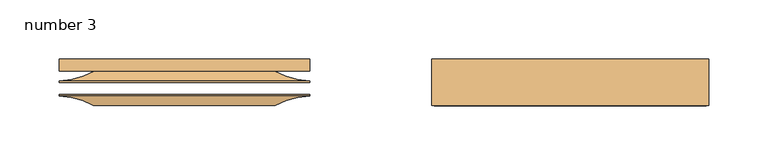
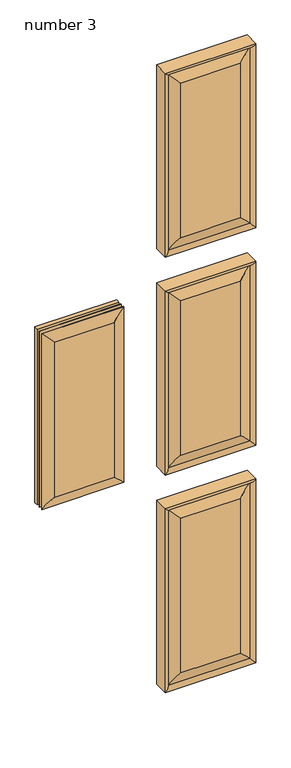
# IFC4 building model written with IfcOpenShell, lengths in millimetres: door geometry, Door-Interior-Karona-K5660-6_Panel : number 3.
# Revit data of these elements (continued)
# Type "Door-Interior-Karona-K5660-6_Panel : number 3" (continued)
#   Bottom Rail Height = 0' - 8 1/2"
#   3D Open Angle = 0.00°
#   Thickness = 0' - 1 3/4"
#   Stop Thickness = 0' - 0 1/2"
#   Stop Depth = 0' - 1 3/8"
#   Rough Width = 2' - 9 29/32"
#   Rough Height = 6' - 8 61/64"
#   Rabbet Width = 0' - 1 3/4"
#   Jamb Offset = 0' - 0 61/64"
#   Hinge Offset = 0' - 0 3/4"
#   Jamb Thickness = 0' - 0 29/32"
#   Ext. Frame Thickness = 0' - 0 5/8"
#   Int. Frame Thickness = 0' - 0 5/8"
#   Height = 6' - 8"
#   Width = 2' - 8"
#   3D Angle = 0.00°
#   Trim Visible = yes
#   Square Sticking Profile = no
#   Raised Panel Door = yes
#   Ovolo Sticking Profile = yes
#   Ogee Sticking Profile = no
#   Mission Sticking Profile = no
#   Hinge Visible = yes
#   Glass Panel Door = no
#   Flat Panel Door = no
#   Edition number = 1
#   Define Thermal Properties by = 1
#   Trim Material = Wood - Karona - Red Oak
#   Top Rail Material = Wood - Karona - Red Oak
#   Stile Material = Wood - Karona - Red Oak
#   Sticking Material = Wood - Karona - Red Oak
#   Jamb Material = Wood - Karona - Red Oak
#   Interior Panel = Wood - Karona - Red Oak
#   Door Panel Material = Wood - Karona - Red Oak
#   Bottom Rail Material = Wood - Karona - Red Oak
#   Visual Light Transmittance = 0
#   Solar Heat Gain Coefficient = 0
#   Construction Type = (empty or 0)
#   Function = (empty or 0)
#   Wall Closure = (empty or 0)
# Element 1 (IfcDoor, "Door-Interior-Karona-K5660-6_Panel : number 3")
#   Materials on its faces: "Wood - Karona - Red Oak"
# Materials
#   "Wood - Karona - Red Oak": class "Wood", colour RGB 153 121 89, transparency 0, Description = "Quercus Rubra", Cost = 0
